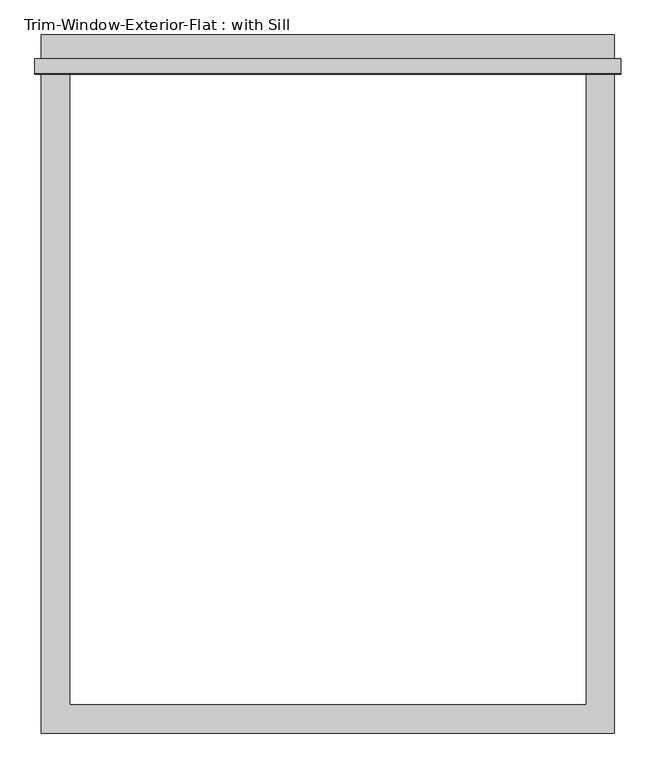
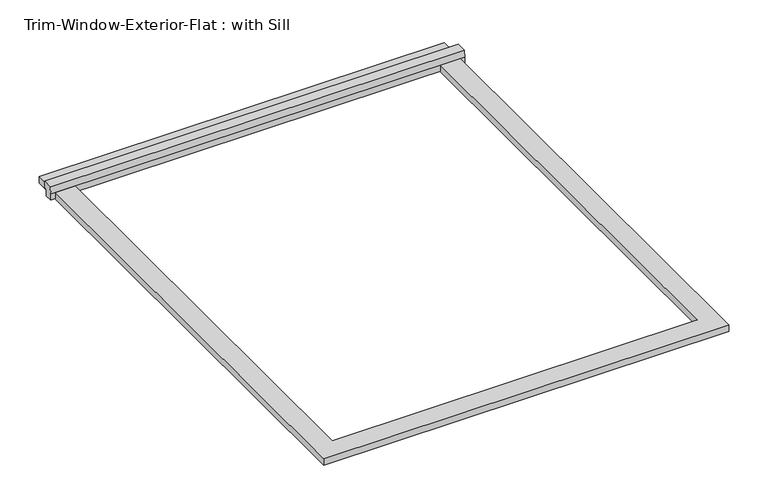
"""IFC4 building model written with IfcOpenShell, lengths in millimetres: proxy geometry, Trim-Window-Exterior-Flat : with Sill."""

from ifc_helpers import new_model, si_unit, frame, origin, origin_with_axes, place, context, project, spatial, polyline, outline, extrude, source, transform, mapped, element, save


def trim_window_exterior_flat_with_sill_256f2652(model_context):
    return source(origin(), model_context, "Body", "SweptSolid", [
        extrude(outline(polyline([(577.85, 1292.1823709), (-577.85, 1292.1823709), (-577.85, 1349.3323709), (577.85, 1349.3323709), (577.85, 1292.1823709)])), origin_with_axes(), (0.0, 0.0, 1.0), 19.05),
        extrude(outline(polyline([(1301.75, 38.1), (1301.75, 19.05), (1292.1823709, 19.05), (1292.1823709, 0.0), (1270.0, 0.0), (1270.0, 19.05), (1272.4580645, 38.1), (1301.75, 38.1)])), frame((-590.55, 0.0, 0.0), z_axis=(1.0, 0.0, 0.0), x_axis=(0.0, 1.0, 0.0)), (0.0, 0.0, 1.0), 1181.1),
        extrude(outline(polyline([(-577.85, -57.15), (-577.85, 1270.0), (-520.7, 1270.0), (-520.7, 0.0), (520.7, 0.0), (520.7, 1270.0), (577.85, 1270.0), (577.85, -57.15), (-577.85, -57.15)])), origin_with_axes(), (0.0, 0.0, 1.0), 19.05),
    ])


if __name__ == "__main__":
    model = new_model("IFC4")
    model_context = context("Model", 3, world=origin())
    ifc_project = project(units=[si_unit("LENGTHUNIT", "METRE", prefix="MILLI")], contexts=[model_context])
    site = spatial("IfcSite", under=ifc_project)
    building = spatial("IfcBuilding", under=site)
    placement = place(None, origin())
    trim_window_exterior_flat_with_sill_shape = trim_window_exterior_flat_with_sill_256f2652(model_context)
    element("IfcBuildingElementProxy", 1, Name="Trim-Window-Exterior-Flat : with Sill", ObjectType="Trim-Window-Exterior-Flat : with Sill", at=placement, inside=building, context=model_context, shape_type="MappedRepresentation", body=[
        mapped(trim_window_exterior_flat_with_sill_shape, transform((0.0, 0.0, 0.0), x_axis=(1.0, 0.0, 0.0), y_axis=(0.0, 1.0, 0.0), z_axis=(0.0, 0.0, 1.0))),
    ])
    save(model, "model.ifc")

# Revit data of these elements
# Type "Trim-Window-Exterior-Flat : with Sill"
#   Trim Width = 0' - 2 1/4"
#   Trim Thickness_Picture Frame = 0' - 1 1/4"
#   Trim Thickness_with Sill = 0' - 0 3/4"
#   Sill Thickness = 0' - 1 1/4"
#   Opening Width [instance default] = 2' - 0"
#   Opening Height [instance default] = 3' - 0"
#   Default Elevation = 4' - 0"
#   Sill = yes
#   Picture Frame = no
#   Trim Material [instance default] = none
# Element 1 (IfcBuildingElementProxy, "Trim-Window-Exterior-Flat : with Sill")
#   Opening Width = 3' - 5"
#   Opening Height = 4' - 2"
#   Trim Material = Clad - White
#   Materials on its faces: "Clad - White"
# Materials
#   "Clad - White": class "Wood", colour RGB 242 242 238, transparency 0, Cost = 0
